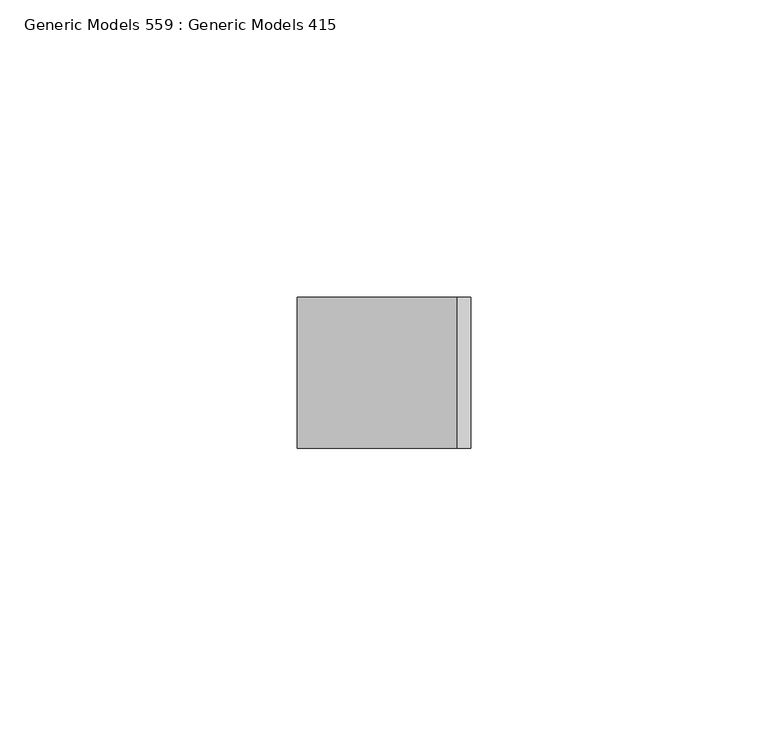
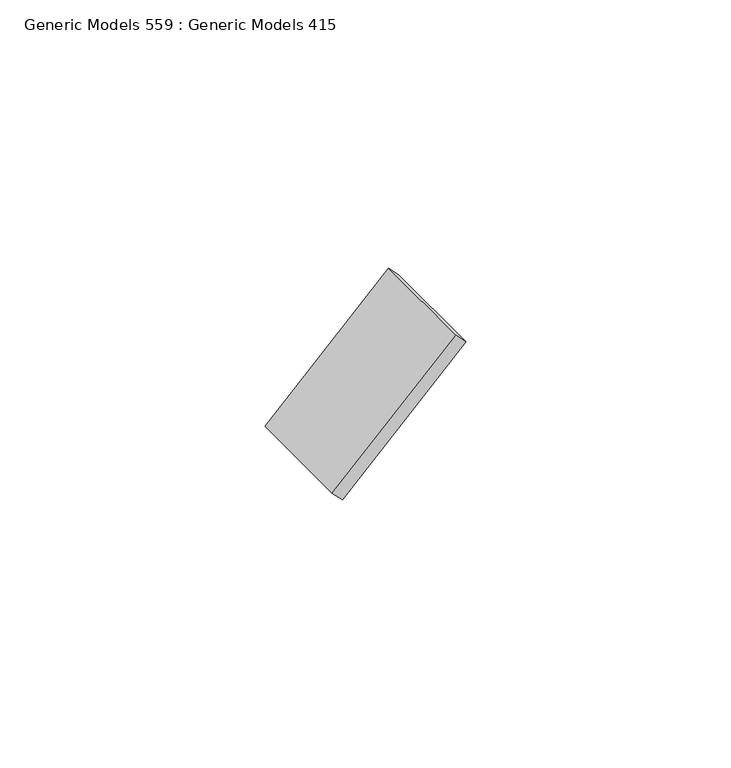
"""IFC4 building model written with IfcOpenShell, lengths in millimetres: proxy geometry, Generic Models 559 : Generic Models 415."""

import ifcopenshell
import ifcopenshell.guid

model = None  # the IFC model being written
_history = None  # IfcOwnerHistory: only IFC2X3 demands one
_inside = {}  # id of a spatial element -> (the spatial element, [elements in it])
_under = {}  # id of a project, library or spatial element -> (it, [spatial elements below it])
_declared = {}  # id of a project -> (the project, [libraries it declares])
_typed = {}  # id of a type object -> (the type object, [elements of that type])
_made_of = {}  # id of a material, layer set ... -> (it, [elements and type objects made of it])


def new_model(schema):
    """Start an empty IFC model of exactly this schema.

    Asked for "IFC4X3", IfcOpenShell would pick the latest addendum, in which some entities
    have other attributes; the version numbers below select the first issue.
    IFC2X3 requires an IfcOwnerHistory on every rooted entity: one is made here for all.
    """
    global model, _history
    if schema == "IFC4X3":
        model = ifcopenshell.file(schema_version=(4, 3, 0, 0))
    else:
        model = ifcopenshell.file(schema=schema)
    _inside.clear()
    _under.clear()
    _declared.clear()
    _typed.clear()
    _made_of.clear()
    _history = None
    if model.schema == "IFC2X3":
        org = make("IfcOrganization", Name="unknown")
        user = make(
            "IfcPersonAndOrganization",
            ThePerson=make("IfcPerson", FamilyName="unknown"),
            TheOrganization=org,
        )
        app = make(
            "IfcApplication",
            ApplicationDeveloper=org,
            Version="unknown",
            ApplicationFullName="unknown",
            ApplicationIdentifier="unknown",
        )
        _history = make(
            "IfcOwnerHistory",
            OwningUser=user,
            OwningApplication=app,
            ChangeAction="ADDED",
            CreationDate=0,
        )
    return model


def make(cls, **values):
    """One entity of the class cls with the attributes given. An attribute that is None is left unset."""
    return model.create_entity(
        cls, **{name: value for name, value in values.items() if value is not None}
    )


def rooted(cls, **values):
    """An entity with a GlobalId (a new one), such as an element, a storey or a relation."""
    return make(cls, GlobalId=ifcopenshell.guid.new(), OwnerHistory=_history, **values)


def si_unit(unit_type, name, prefix=None):
    """IfcSIUnit, for example si_unit("LENGTHUNIT", "METRE", prefix="MILLI")."""
    return make("IfcSIUnit", UnitType=unit_type, Prefix=prefix, Name=name)


def assignment(units):
    """IfcUnitAssignment: the units of a project."""
    return None if units is None else make("IfcUnitAssignment", Units=units)


def point(xyz):
    """IfcCartesianPoint."""
    return None if xyz is None else make("IfcCartesianPoint", Coordinates=xyz)


def direction(xyz):
    """IfcDirection."""
    return None if xyz is None else make("IfcDirection", DirectionRatios=xyz)


def frame(location, z_axis=None, x_axis=None):
    """IfcAxis2Placement3D, a coordinate frame: its origin and axes. An axis left out is left unset."""
    return make(
        "IfcAxis2Placement3D",
        Location=point(location),
        Axis=direction(z_axis),
        RefDirection=direction(x_axis),
    )


def origin():
    """The frame at (0, 0, 0) with its axes left unset."""
    return frame((0.0, 0.0, 0.0))


def place(relative_to, where):
    """IfcLocalPlacement: puts the frame where relative to a parent placement (None: the world)."""
    return make(
        "IfcLocalPlacement", PlacementRelTo=relative_to, RelativePlacement=where
    )


def context(
    kind, dimensions, precision=None, world=None, true_north=None, identifier=None
):
    """IfcGeometricRepresentationContext, for example the 3D "Model" context."""
    return make(
        "IfcGeometricRepresentationContext",
        ContextIdentifier=identifier,
        ContextType=kind,
        CoordinateSpaceDimension=dimensions,
        Precision=precision,
        WorldCoordinateSystem=world,
        TrueNorth=true_north,
    )


def project(units=None, contexts=None):
    """IfcProject with its units and contexts."""
    return rooted(
        "IfcProject",
        Name="project",
        RepresentationContexts=contexts,
        UnitsInContext=assignment(units),
    )


def spatial(cls, under=None, at=None, **own):
    """A site, building, storey or space (cls), placed at a placement, below another one or the project."""
    s = rooted(cls, ObjectPlacement=at, **own)
    if under is not None:
        _under.setdefault(under.id(), (under, []))[1].append(s)
    return s


def polyline(points):
    """IfcPolyline through the points."""
    return make("IfcPolyline", Points=[point(p) for p in points])


def outline(outer, holes=None, kind="AREA"):
    """IfcArbitraryClosedProfileDef: a profile drawn as a closed curve; with holes, ...WithVoids."""
    if holes is None:
        return make("IfcArbitraryClosedProfileDef", ProfileType=kind, OuterCurve=outer)
    return make(
        "IfcArbitraryProfileDefWithVoids",
        ProfileType=kind,
        OuterCurve=outer,
        InnerCurves=holes,
    )


def extrude(swept, where, along, depth):
    """IfcExtrudedAreaSolid: the profile swept, set in the frame where, extruded along a direction by depth."""
    return make(
        "IfcExtrudedAreaSolid",
        SweptArea=swept,
        Position=where,
        ExtrudedDirection=direction(along),
        Depth=depth,
    )


def shape(context_of_items, identifier, shape_type, items):
    """IfcShapeRepresentation: the items that make up one representation, for example the "Body"."""
    return make(
        "IfcShapeRepresentation",
        ContextOfItems=context_of_items,
        RepresentationIdentifier=identifier,
        RepresentationType=shape_type,
        Items=items,
    )


def source(mapping_origin, context_of_items, identifier, shape_type, items):
    """IfcRepresentationMap: a shape defined once, which mapped items show again and again."""
    return make(
        "IfcRepresentationMap",
        MappingOrigin=mapping_origin,
        MappedRepresentation=shape(context_of_items, identifier, shape_type, items),
    )


def transform(
    local_origin,
    x_axis=None,
    y_axis=None,
    z_axis=None,
    scale=None,
    scale2=None,
    scale3=None,
    uniform=True,
):
    """IfcCartesianTransformationOperator3D, or its non-uniform kind. x_axis, y_axis, z_axis: its Axis1, 2, 3."""
    if uniform:
        return make(
            "IfcCartesianTransformationOperator3D",
            Axis1=direction(x_axis),
            Axis2=direction(y_axis),
            LocalOrigin=point(local_origin),
            Scale=scale,
            Axis3=direction(z_axis),
        )
    return make(
        "IfcCartesianTransformationOperator3DnonUniform",
        Axis1=direction(x_axis),
        Axis2=direction(y_axis),
        LocalOrigin=point(local_origin),
        Scale=scale,
        Axis3=direction(z_axis),
        Scale2=scale2,
        Scale3=scale3,
    )


def mapped(mapping_source, mapping_target):
    """IfcMappedItem: shows the shape of a source again, moved by a transform."""
    return make(
        "IfcMappedItem", MappingSource=mapping_source, MappingTarget=mapping_target
    )


def made_of(thing, what):
    """Note that an element or type object is made of a material, layer set ...; save() writes the relation."""
    if what is not None:
        _made_of.setdefault(what.id(), (what, []))[1].append(thing)
    return thing


def element(
    cls,
    number,
    at=None,
    inside=None,
    cuts=None,
    type_object=None,
    material=None,
    context=None,
    identifier="Body",
    shape_type=None,
    held_by="IfcProductDefinitionShape",
    body=None,
    shapes=None,
    **own,
):
    """One element of the class cls, such as IfcWall. Its Tag is "e" and its number.

    at: its placement. inside: the storey or other place that contains it. cuts: it is an
    opening in that element (IfcRelVoidsElement). A single representation is given by context,
    identifier, shape_type and body (its items); several are given by shapes. held_by: the class
    of the entity that holds the representations. save() writes the other relations.
    """
    e = rooted(cls, Tag="e%d" % number, ObjectPlacement=at, **own)
    if body is not None:
        shapes = [shape(context, identifier, shape_type, body)]
    if shapes is not None:
        e.Representation = make(held_by, Representations=shapes)
    if inside is not None:
        _inside.setdefault(inside.id(), (inside, []))[1].append(e)
    if cuts is not None:
        rooted(
            "IfcRelVoidsElement", RelatingBuildingElement=cuts, RelatedOpeningElement=e
        )
    if type_object is not None:
        _typed.setdefault(type_object.id(), (type_object, []))[1].append(e)
    return made_of(e, material)


def aggregate(whole, parts):
    """IfcRelAggregates: a whole, such as a stair, and the parts it consists of."""
    return rooted("IfcRelAggregates", RelatingObject=whole, RelatedObjects=parts)


def save(model, path):
    """Write the relations noted so far, then the file.

    IfcRelAggregates (storeys below a building ...), IfcRelContainedInSpatialStructure (elements
    in a storey), IfcRelDefinesByType, IfcRelAssociatesMaterial and IfcRelDeclares: one each for
    every whole, place, type object, material and project.
    """
    for whole, parts in _under.values():
        aggregate(whole, parts)
    for where, things in _inside.values():
        rooted(
            "IfcRelContainedInSpatialStructure",
            RelatedElements=things,
            RelatingStructure=where,
        )
    for kind, things in _typed.values():
        rooted("IfcRelDefinesByType", RelatedObjects=things, RelatingType=kind)
    for what, things in _made_of.values():
        rooted("IfcRelAssociatesMaterial", RelatedObjects=things, RelatingMaterial=what)
    for by, libraries in _declared.values():
        rooted("IfcRelDeclares", RelatingContext=by, RelatedDefinitions=libraries)
    model.write(path)


def generic_models_559_generic_models_415_af826ab2(model_context):
    return source(origin(), model_context, "Body", "SweptSolid", [
        extrude(outline(polyline([(0.0, -3.175), (0.0, 0.0), (25.4, 0.0), (25.4, -3.175), (0.0, -3.175)])), frame((7848.0411784, 4501.3863946, 124432.3849742), z_axis=(0.7071067811867181, 0.0, 0.707106781186377), x_axis=(0.0, -1.0, 0.0)), (0.0, 0.0, 1.0), 38.1),
    ])


if __name__ == "__main__":
    model = new_model("IFC4")
    model_context = context("Model", 3, world=origin())
    ifc_project = project(units=[si_unit("LENGTHUNIT", "METRE", prefix="MILLI")], contexts=[model_context])
    site = spatial("IfcSite", under=ifc_project)
    building = spatial("IfcBuilding", under=site)
    placement = place(None, origin())
    generic_models_559_generic_models_415_shape = generic_models_559_generic_models_415_af826ab2(model_context)
    element("IfcBuildingElementProxy", 1, Name="Generic Models 559 : Generic Models 415", ObjectType="Generic Models 559 : Generic Models 415", at=placement, inside=building, context=model_context, shape_type="MappedRepresentation", body=[
        mapped(generic_models_559_generic_models_415_shape, transform((0.0, 0.0, 0.0), x_axis=(1.0, 0.0, 0.0), y_axis=(0.0, 1.0, 0.0), z_axis=(0.0, 0.0, 1.0))),
    ])
    save(model, "model.ifc")

# Revit data of these elements
# Element 1 (IfcBuildingElementProxy, "Generic Models 559 : Generic Models 415")
#   Materials on its faces: "_WELDED STEEL TABS FOR LOUVER ATTACHMENT"
# Materials
#   "_WELDED STEEL TABS FOR LOUVER ATTACHMENT": class "Metal", colour RGB 199 199 199, transparency 0, Description = "Structural steel 50ksi", Cost = 0
